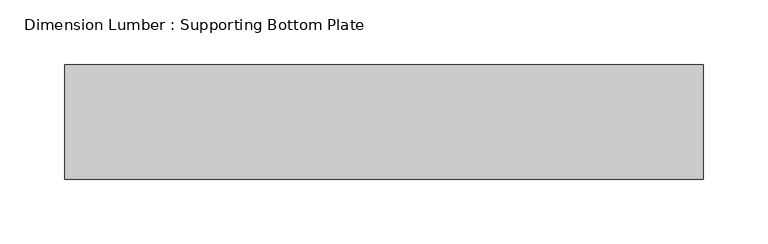
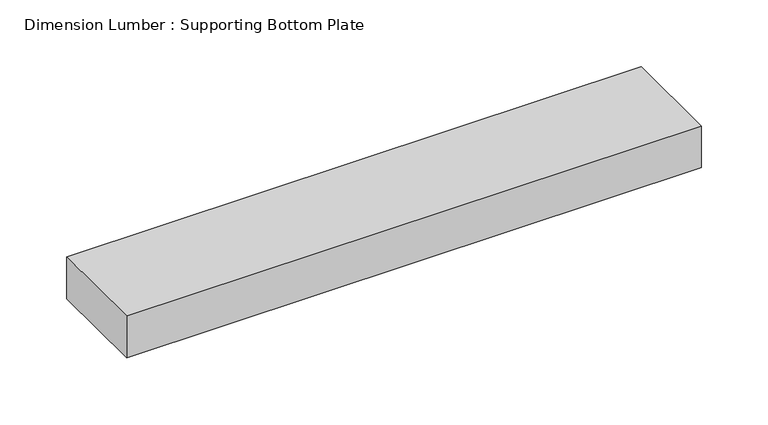
"""IFC4 building model written with IfcOpenShell, lengths in millimetres: beam geometry, Dimension Lumber : Supporting Bottom Plate."""

from ifc_helpers import new_model, si_unit, frame, origin, place, context, project, spatial, polyline, outline, extrude, source, transform, mapped, element, save


def dimension_lumber_supporting_bottom_plate_47a8c852(model_context):
    return source(origin(), model_context, "Body", "SweptSolid", [
        extrude(outline(polyline([(292.0, 44.45), (292.0, -44.45), (-203.1, -44.45), (-203.1, 44.45), (292.0, 44.45)])), frame((0.0, 0.0, -19.05), z_axis=(0.0, 0.0, 1.0), x_axis=(1.0, 0.0, 0.0)), (0.0, 0.0, 1.0), 38.1),
    ])


if __name__ == "__main__":
    model = new_model("IFC4")
    model_context = context("Model", 3, world=origin())
    ifc_project = project(units=[si_unit("LENGTHUNIT", "METRE", prefix="MILLI")], contexts=[model_context])
    site = spatial("IfcSite", under=ifc_project)
    building = spatial("IfcBuilding", under=site)
    placement = place(None, origin())
    dimension_lumber_supporting_bottom_plate_shape = dimension_lumber_supporting_bottom_plate_47a8c852(model_context)
    element("IfcBeam", 1, ObjectType="Dimension Lumber : Supporting Bottom Plate", at=placement, inside=building, context=model_context, shape_type="MappedRepresentation", body=[
        mapped(dimension_lumber_supporting_bottom_plate_shape, transform((0.0, 0.0, 0.0), x_axis=(1.0, 0.0, 0.0), y_axis=(0.0, 1.0, 0.0), z_axis=(0.0, 0.0, 1.0))),
    ])
    save(model, "model.ifc")

# Revit data of these elements
# Type "Dimension Lumber : Supporting Bottom Plate"
#   Assembly Code = "B10"
#   A = 0.0364583 SF
#   Length [instance default] = 5' - 0"
#   b = 0' - 3 1/2"
#   d = 0' - 1 1/2"
#   Structural Material [instance default] = Softwood, Lumber
# Element 1 (IfcBeam, "Dimension Lumber : Supporting Bottom Plate")
#   Structural Material = Douglas Fir #2
#   Materials on its faces: "Douglas Fir #2"
# Materials
#   "Softwood, Lumber": class "Wood", colour RGB 223 192 134, transparency 0, Description = "Pinus Echinata", Cost = 0
#   "Douglas Fir #2": class "Wood", colour RGB 223 192 134, transparency 0, Description = "Pinus Echinata", Cost = 0
